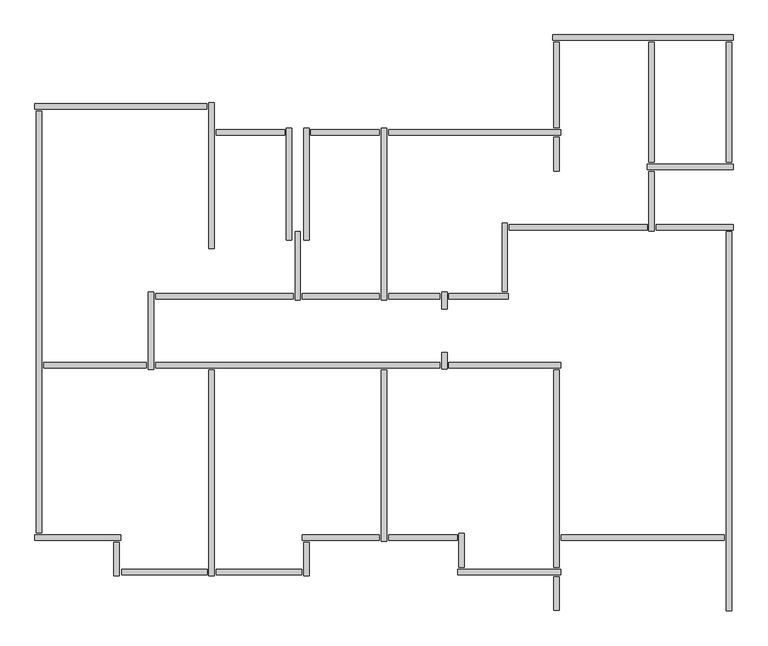
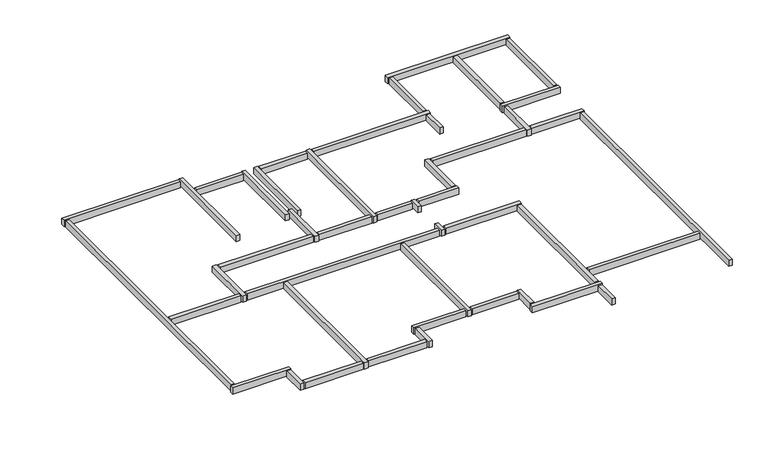
"""IFC4 building model written with IfcOpenShell, lengths in millimetres: beam geometry, Graute viga de respaldo6 : Graute viga de respaldo."""

from ifc_helpers import new_model, si_unit, frame, origin, place, context, project, spatial, polyline, outline, extrude, source, transform, mapped, element, save


def beam_72c07302(model_context):
    return source(origin(), model_context, "Body", "SweptSolid", [
        extrude(outline(polyline([(-75401.7587292, 57502.4278788), (-75401.7587292, 57408.4278788), (-76591.7587292, 57408.4278788), (-76591.7587292, 57502.4278788), (-75401.7587292, 57502.4278788)])), frame((0.0, 0.0, 5632.9999999), z_axis=(0.0, 0.0, 1.0), x_axis=(1.0, 0.0, 0.0)), (0.0, 0.0, 1.0), 167.0),
        extrude(outline(polyline([(-73751.7587292, 57502.4278788), (-73751.7587292, 57408.4278788), (-74941.7587292, 57408.4278788), (-74941.7587292, 57502.4278788), (-73751.7587292, 57502.4278788)])), frame((0.0, 0.0, 5632.9999999), z_axis=(0.0, 0.0, 1.0), x_axis=(1.0, 0.0, 0.0)), (0.0, 0.0, 1.0), 167.0),
        extrude(outline(polyline([(-77801.7587292, 53452.4278788), (-77801.7587292, 53358.4278788), (-79591.7587292, 53358.4278788), (-79591.7587292, 53452.4278788), (-77801.7587292, 53452.4278788)])), frame((0.0, 0.0, 5632.9999999), z_axis=(0.0, 0.0, 1.0), x_axis=(1.0, 0.0, 0.0)), (0.0, 0.0, 1.0), 167.0),
        extrude(outline(polyline([(-72401.7587292, 50452.4278788), (-72401.7587292, 50358.4278788), (-73591.7587292, 50358.4278788), (-73591.7587292, 50452.4278788), (-72401.7587292, 50452.4278788)])), frame((0.0, 0.0, 5632.9999999), z_axis=(0.0, 0.0, 1.0), x_axis=(1.0, 0.0, 0.0)), (0.0, 0.0, 1.0), 167.0),
        extrude(outline(polyline([(-72368.7587292, 50475.4278788), (-72274.7587292, 50475.4278788), (-72274.7587292, 49885.4278788), (-72368.7587292, 49885.4278788), (-72368.7587292, 50475.4278788)])), frame((0.0, 0.0, 5632.9999999), z_axis=(0.0, 0.0, 1.0), x_axis=(1.0, 0.0, 0.0)), (0.0, 0.0, 1.0), 167.0),
        extrude(outline(polyline([(-70601.7587292, 49852.4278788), (-70601.7587292, 49758.4278788), (-72391.7587292, 49758.4278788), (-72391.7587292, 49852.4278788), (-70601.7587292, 49852.4278788)])), frame((0.0, 0.0, 5632.9999999), z_axis=(0.0, 0.0, 1.0), x_axis=(1.0, 0.0, 0.0)), (0.0, 0.0, 1.0), 167.0),
        extrude(outline(polyline([(-72574.7587292, 53335.4278788), (-72668.7587292, 53335.4278788), (-72668.7587292, 53625.4278788), (-72574.7587292, 53625.4278788), (-72574.7587292, 53335.4278788)])), frame((0.0, 0.0, 5632.9999999), z_axis=(0.0, 0.0, 1.0), x_axis=(1.0, 0.0, 0.0)), (0.0, 0.0, 1.0), 167.0),
        extrude(outline(polyline([(-75251.7587292, 54652.4278788), (-75251.7587292, 54558.4278788), (-77641.7587292, 54558.4278788), (-77641.7587292, 54652.4278788), (-75251.7587292, 54652.4278788)])), frame((0.0, 0.0, 5632.9999999), z_axis=(0.0, 0.0, 1.0), x_axis=(1.0, 0.0, 0.0)), (0.0, 0.0, 1.0), 167.0),
        extrude(outline(polyline([(-73751.7587292, 54652.4278788), (-73751.7587292, 54558.4278788), (-75091.7587292, 54558.4278788), (-75091.7587292, 54652.4278788), (-73751.7587292, 54652.4278788)])), frame((0.0, 0.0, 5632.9999999), z_axis=(0.0, 0.0, 1.0), x_axis=(1.0, 0.0, 0.0)), (0.0, 0.0, 1.0), 167.0),
        extrude(outline(polyline([(-72701.7587292, 54652.4278788), (-72701.7587292, 54558.4278788), (-73591.7587292, 54558.4278788), (-73591.7587292, 54652.4278788), (-72701.7587292, 54652.4278788)])), frame((0.0, 0.0, 5632.9999999), z_axis=(0.0, 0.0, 1.0), x_axis=(1.0, 0.0, 0.0)), (0.0, 0.0, 1.0), 167.0),
        extrude(outline(polyline([(-72574.7587292, 54385.4278788), (-72668.7587292, 54385.4278788), (-72668.7587292, 54675.4278788), (-72574.7587292, 54675.4278788), (-72574.7587292, 54385.4278788)])), frame((0.0, 0.0, 5632.9999999), z_axis=(0.0, 0.0, 1.0), x_axis=(1.0, 0.0, 0.0)), (0.0, 0.0, 1.0), 167.0),
        extrude(outline(polyline([(-71511.7587292, 54652.4278788), (-71511.7587292, 54558.4278788), (-72541.7587292, 54558.4278788), (-72541.7587292, 54652.4278788), (-71511.7587292, 54652.4278788)])), frame((0.0, 0.0, 5632.9999999), z_axis=(0.0, 0.0, 1.0), x_axis=(1.0, 0.0, 0.0)), (0.0, 0.0, 1.0), 167.0),
        extrude(outline(polyline([(-71618.7587292, 55875.4278788), (-71524.7587292, 55875.4278788), (-71524.7587292, 54685.4278788), (-71618.7587292, 54685.4278788), (-71618.7587292, 55875.4278788)])), frame((0.0, 0.0, 5632.9999999), z_axis=(0.0, 0.0, 1.0), x_axis=(1.0, 0.0, 0.0)), (0.0, 0.0, 1.0), 167.0),
        extrude(outline(polyline([(-69091.7587292, 55852.4278788), (-69091.7587292, 55758.4278788), (-71491.7587292, 55758.4278788), (-71491.7587292, 55852.4278788), (-69091.7587292, 55852.4278788)])), frame((0.0, 0.0, 5632.9999999), z_axis=(0.0, 0.0, 1.0), x_axis=(1.0, 0.0, 0.0)), (0.0, 0.0, 1.0), 167.0),
        extrude(outline(polyline([(-73624.7587292, 54540.4278788), (-73718.7587292, 54540.4278788), (-73718.7587292, 57525.4278788), (-73624.7587292, 57525.4278788), (-73624.7587292, 54540.4278788)])), frame((0.0, 0.0, 5632.9999999), z_axis=(0.0, 0.0, 1.0), x_axis=(1.0, 0.0, 0.0)), (0.0, 0.0, 1.0), 167.0),
        extrude(outline(polyline([(-70601.7587292, 57502.4278788), (-70601.7587292, 57408.4278788), (-73591.7587292, 57408.4278788), (-73591.7587292, 57502.4278788), (-70601.7587292, 57502.4278788)])), frame((0.0, 0.0, 5632.9999999), z_axis=(0.0, 0.0, 1.0), x_axis=(1.0, 0.0, 0.0)), (0.0, 0.0, 1.0), 167.0),
        extrude(outline(polyline([(-70624.7587292, 56785.4278788), (-70718.7587292, 56785.4278788), (-70718.7587292, 57375.4278788), (-70624.7587292, 57375.4278788), (-70624.7587292, 56785.4278788)])), frame((0.0, 0.0, 5632.9999999), z_axis=(0.0, 0.0, 1.0), x_axis=(1.0, 0.0, 0.0)), (0.0, 0.0, 1.0), 167.0),
        extrude(outline(polyline([(-70718.7587292, 59025.4278788), (-70624.7587292, 59025.4278788), (-70624.7587292, 57535.4278788), (-70718.7587292, 57535.4278788), (-70718.7587292, 59025.4278788)])), frame((0.0, 0.0, 5632.9999999), z_axis=(0.0, 0.0, 1.0), x_axis=(1.0, 0.0, 0.0)), (0.0, 0.0, 1.0), 167.0),
        extrude(outline(polyline([(-67718.7587292, 59025.4278788), (-67624.7587292, 59025.4278788), (-67624.7587292, 56935.4278788), (-67718.7587292, 56935.4278788), (-67718.7587292, 59025.4278788)])), frame((0.0, 0.0, 5632.9999999), z_axis=(0.0, 0.0, 1.0), x_axis=(1.0, 0.0, 0.0)), (0.0, 0.0, 1.0), 167.0),
        extrude(outline(polyline([(-69068.7587292, 59025.4278788), (-68974.7587292, 59025.4278788), (-68974.7587292, 56935.4278788), (-69068.7587292, 56935.4278788), (-69068.7587292, 59025.4278788)])), frame((0.0, 0.0, 5632.9999999), z_axis=(0.0, 0.0, 1.0), x_axis=(1.0, 0.0, 0.0)), (0.0, 0.0, 1.0), 167.0),
        extrude(outline(polyline([(-68974.7587292, 55735.4278788), (-69068.7587292, 55735.4278788), (-69068.7587292, 56775.4278788), (-68974.7587292, 56775.4278788), (-68974.7587292, 55735.4278788)])), frame((0.0, 0.0, 5632.9999999), z_axis=(0.0, 0.0, 1.0), x_axis=(1.0, 0.0, 0.0)), (0.0, 0.0, 1.0), 167.0),
        extrude(outline(polyline([(-67751.7587292, 50452.4278788), (-67751.7587292, 50358.4278788), (-70591.7587292, 50358.4278788), (-70591.7587292, 50452.4278788), (-67751.7587292, 50452.4278788)])), frame((0.0, 0.0, 5632.9999999), z_axis=(0.0, 0.0, 1.0), x_axis=(1.0, 0.0, 0.0)), (0.0, 0.0, 1.0), 167.0),
        extrude(outline(polyline([(-70718.7587292, 53325.4278788), (-70624.7587292, 53325.4278788), (-70624.7587292, 49885.4278788), (-70718.7587292, 49885.4278788), (-70718.7587292, 53325.4278788)])), frame((0.0, 0.0, 5632.9999999), z_axis=(0.0, 0.0, 1.0), x_axis=(1.0, 0.0, 0.0)), (0.0, 0.0, 1.0), 167.0),
        extrude(outline(polyline([(-70601.7587292, 53452.4278788), (-70601.7587292, 53358.4278788), (-72541.7587292, 53358.4278788), (-72541.7587292, 53452.4278788), (-70601.7587292, 53452.4278788)])), frame((0.0, 0.0, 5632.9999999), z_axis=(0.0, 0.0, 1.0), x_axis=(1.0, 0.0, 0.0)), (0.0, 0.0, 1.0), 167.0),
        extrude(outline(polyline([(-72701.7587292, 53452.4278788), (-72701.7587292, 53358.4278788), (-77641.7587292, 53358.4278788), (-77641.7587292, 53452.4278788), (-72701.7587292, 53452.4278788)])), frame((0.0, 0.0, 5632.9999999), z_axis=(0.0, 0.0, 1.0), x_axis=(1.0, 0.0, 0.0)), (0.0, 0.0, 1.0), 167.0),
        extrude(outline(polyline([(-73624.7587292, 50335.4278788), (-73718.7587292, 50335.4278788), (-73718.7587292, 53325.4278788), (-73624.7587292, 53325.4278788), (-73624.7587292, 50335.4278788)])), frame((0.0, 0.0, 5632.9999999), z_axis=(0.0, 0.0, 1.0), x_axis=(1.0, 0.0, 0.0)), (0.0, 0.0, 1.0), 167.0),
        extrude(outline(polyline([(-75091.7587292, 50358.4278788), (-75091.7587292, 50452.4278788), (-73751.7587292, 50452.4278788), (-73751.7587292, 50358.4278788), (-75091.7587292, 50358.4278788)])), frame((0.0, 0.0, 5632.9999999), z_axis=(0.0, 0.0, 1.0), x_axis=(1.0, 0.0, 0.0)), (0.0, 0.0, 1.0), 167.0),
        extrude(outline(polyline([(-74974.7587292, 49735.4278788), (-75068.7587292, 49735.4278788), (-75068.7587292, 50325.4278788), (-74974.7587292, 50325.4278788), (-74974.7587292, 49735.4278788)])), frame((0.0, 0.0, 5632.9999999), z_axis=(0.0, 0.0, 1.0), x_axis=(1.0, 0.0, 0.0)), (0.0, 0.0, 1.0), 167.0),
        extrude(outline(polyline([(-75101.7587292, 49852.4278788), (-75101.7587292, 49758.4278788), (-76591.7587292, 49758.4278788), (-76591.7587292, 49852.4278788), (-75101.7587292, 49852.4278788)])), frame((0.0, 0.0, 5632.9999999), z_axis=(0.0, 0.0, 1.0), x_axis=(1.0, 0.0, 0.0)), (0.0, 0.0, 1.0), 167.0),
        extrude(outline(polyline([(-78230.736554, 49758.4278788), (-78230.736554, 49853.4278788), (-76741.7587292, 49853.4278788), (-76741.7587292, 49758.4278788), (-78230.736554, 49758.4278788)])), frame((0.0, 0.0, 5617.1856208), z_axis=(0.0, 0.0, 1.0), x_axis=(1.0, 0.0, 0.0)), (0.0, 0.0, 1.0), 165.0),
        extrude(outline(polyline([(-79718.7587292, 57825.4278788), (-79624.7587292, 57825.4278788), (-79624.7587292, 50485.4278788), (-79718.7587292, 50485.4278788), (-79718.7587292, 57825.4278788)])), frame((0.0, 0.0, 5632.9999999), z_axis=(0.0, 0.0, 1.0), x_axis=(1.0, 0.0, 0.0)), (0.0, 0.0, 1.0), 167.0),
        extrude(outline(polyline([(-77768.7587292, 54675.4278788), (-77674.7587292, 54675.4278788), (-77674.7587292, 53330.0746661), (-77768.7587292, 53330.0746661), (-77768.7587292, 54675.4278788)])), frame((0.0, 0.0, 5632.9999999), z_axis=(0.0, 0.0, 1.0), x_axis=(1.0, 0.0, 0.0)), (0.0, 0.0, 1.0), 167.0),
        extrude(outline(polyline([(-75218.7587292, 55725.4278788), (-75124.7587292, 55725.4278788), (-75124.7587292, 54535.4278788), (-75218.7587292, 54535.4278788), (-75218.7587292, 55725.4278788)])), frame((0.0, 0.0, 5632.9999999), z_axis=(0.0, 0.0, 1.0), x_axis=(1.0, 0.0, 0.0)), (0.0, 0.0, 1.0), 167.0),
        extrude(outline(polyline([(-75368.7587292, 57525.4278788), (-75274.7587292, 57525.4278788), (-75274.7587292, 55585.4278788), (-75368.7587292, 55585.4278788), (-75368.7587292, 57525.4278788)])), frame((0.0, 0.0, 5632.9999999), z_axis=(0.0, 0.0, 1.0), x_axis=(1.0, 0.0, 0.0)), (0.0, 0.0, 1.0), 167.0),
        extrude(outline(polyline([(-75068.7587292, 57525.4278788), (-74974.7587292, 57525.4278788), (-74974.7587292, 55585.4278788), (-75068.7587292, 55585.4278788), (-75068.7587292, 57525.4278788)])), frame((0.0, 0.0, 5632.9999999), z_axis=(0.0, 0.0, 1.0), x_axis=(1.0, 0.0, 0.0)), (0.0, 0.0, 1.0), 167.0),
        extrude(outline(polyline([(-76718.7587292, 57975.4278788), (-76624.7587292, 57975.4278788), (-76624.7587292, 55435.4278788), (-76718.7587292, 55435.4278788), (-76718.7587292, 57975.4278788)])), frame((0.0, 0.0, 5632.9999999), z_axis=(0.0, 0.0, 1.0), x_axis=(1.0, 0.0, 0.0)), (0.0, 0.0, 1.0), 167.0),
        extrude(outline(polyline([(-79741.7587292, 57858.4278788), (-79741.7587292, 57952.4278788), (-76751.7587292, 57952.4278788), (-76751.7587292, 57858.4278788), (-79741.7587292, 57858.4278788)])), frame((0.0, 0.0, 5632.9999999), z_axis=(0.0, 0.0, 1.0), x_axis=(1.0, 0.0, 0.0)), (0.0, 0.0, 1.0), 167.0),
        extrude(outline(polyline([(-78274.7587292, 49735.4278788), (-78368.7587292, 49735.4278788), (-78368.7587292, 50325.4278788), (-78274.7587292, 50325.4278788), (-78274.7587292, 49735.4278788)])), frame((0.0, 0.0, 5632.9999999), z_axis=(0.0, 0.0, 1.0), x_axis=(1.0, 0.0, 0.0)), (0.0, 0.0, 1.0), 167.0),
        extrude(outline(polyline([(-78251.7587292, 50452.4278788), (-78251.7587292, 50358.4278788), (-79741.7587292, 50358.4278788), (-79741.7587292, 50452.4278788), (-78251.7587292, 50452.4278788)])), frame((0.0, 0.0, 5632.9999999), z_axis=(0.0, 0.0, 1.0), x_axis=(1.0, 0.0, 0.0)), (0.0, 0.0, 1.0), 167.0),
        extrude(outline(polyline([(-76624.7587292, 49735.4278788), (-76718.7587292, 49735.4278788), (-76718.7587292, 53325.4278788), (-76624.7587292, 53325.4278788), (-76624.7587292, 49735.4278788)])), frame((0.0, 0.0, 5632.9999999), z_axis=(0.0, 0.0, 1.0), x_axis=(1.0, 0.0, 0.0)), (0.0, 0.0, 1.0), 167.0),
        extrude(outline(polyline([(-70624.7587292, 49135.4278788), (-70718.7587292, 49135.4278788), (-70718.7587292, 49725.4278788), (-70624.7587292, 49725.4278788), (-70624.7587292, 49135.4278788)])), frame((0.0, 0.0, 5632.9999999), z_axis=(0.0, 0.0, 1.0), x_axis=(1.0, 0.0, 0.0)), (0.0, 0.0, 1.0), 167.0),
        extrude(outline(polyline([(-67601.7587292, 56902.4278788), (-67601.7587292, 56808.4278788), (-69091.7587292, 56808.4278788), (-69091.7587292, 56902.4278788), (-67601.7587292, 56902.4278788)])), frame((0.0, 0.0, 5632.9999999), z_axis=(0.0, 0.0, 1.0), x_axis=(1.0, 0.0, 0.0)), (0.0, 0.0, 1.0), 167.0),
        extrude(outline(polyline([(-67601.7587292, 59152.4278788), (-67601.7587292, 59058.4278788), (-70741.7587292, 59058.4278788), (-70741.7587292, 59152.4278788), (-67601.7587292, 59152.4278788)])), frame((0.0, 0.0, 5632.9999999), z_axis=(0.0, 0.0, 1.0), x_axis=(1.0, 0.0, 0.0)), (0.0, 0.0, 1.0), 167.0),
        extrude(outline(polyline([(-67601.7587292, 55852.4278788), (-67601.7587292, 55758.4278788), (-68941.7587292, 55758.4278788), (-68941.7587292, 55852.4278788), (-67601.7587292, 55852.4278788)])), frame((0.0, 0.0, 5632.9999999), z_axis=(0.0, 0.0, 1.0), x_axis=(1.0, 0.0, 0.0)), (0.0, 0.0, 1.0), 167.0),
        extrude(outline(polyline([(-67624.7587292, 49132.8979841), (-67718.7587292, 49132.8979841), (-67718.7587292, 55725.4278788), (-67624.7587292, 55725.4278788), (-67624.7587292, 49132.8979841)])), frame((0.0, 0.0, 5632.9999999), z_axis=(0.0, 0.0, 1.0), x_axis=(1.0, 0.0, 0.0)), (0.0, 0.0, 1.0), 167.0),
    ])


if __name__ == "__main__":
    model = new_model("IFC4")
    model_context = context("Model", 3, world=origin())
    ifc_project = project(units=[si_unit("LENGTHUNIT", "METRE", prefix="MILLI")], contexts=[model_context])
    site = spatial("IfcSite", under=ifc_project)
    building = spatial("IfcBuilding", under=site)
    placement = place(None, origin())
    beam_shape = beam_72c07302(model_context)
    element("IfcBeam", 1, ObjectType="Graute viga de respaldo6 : Graute viga de respaldo", at=placement, inside=building, context=model_context, shape_type="MappedRepresentation", body=[
        mapped(beam_shape, transform((0.0, 0.0, 0.0), x_axis=(1.0, 0.0, 0.0), y_axis=(0.0, 1.0, 0.0), z_axis=(0.0, 0.0, 1.0))),
    ])
    save(model, "model.ifc")

# Revit data of these elements
# Element 1 (IfcBeam, "Graute viga de respaldo6 : Graute viga de respaldo")
#   Materials on its faces: "Concreto, Faixa de areia/cimento"
# Materials
#   "Concreto, Faixa de areia/cimento": class "Concreto", colour RGB 127 127 127, transparency 0, Description = "Revestimento de laje de concreto", Cost = 0
